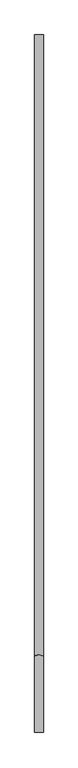
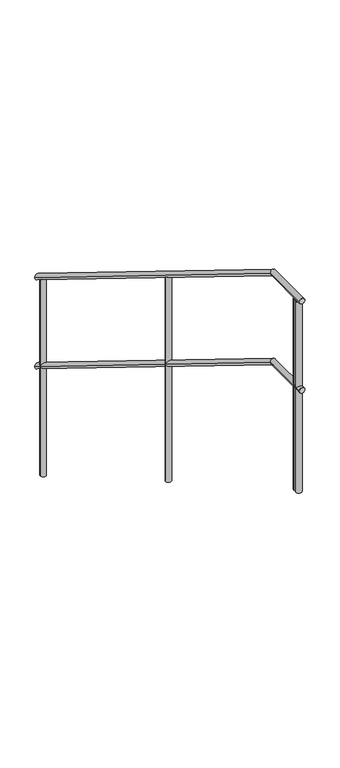
"""IFC4 building model written with IfcOpenShell, lengths in millimetres: railing geometry."""

from ifc_helpers import new_model, si_unit, point, frame, frame_2d, origin, place, context, project, spatial, circle_curve, ellipse_curve, trimmed, segment, composite_curve, outline, extrude, source, transform, mapped, element, save
from ifc_brep_helpers import plane_surface, cylinder_surface, advanced_brep


def railing_fdf8c7c9(model_context):
    return source(origin(), model_context, "Body", "SolidModel", [
        advanced_brep(
        [(-2206.0, 35476.2934796, -450.9609787), (-2176.0, 35476.2934796, -450.9609787), (-2176.0, 33312.0366941, 885.0), (-2206.0, 33312.0366941, 885.0), (-2206.0, 33046.2934796, 885.0), (-2176.0, 33046.2934796, 885.0)],
        [
            (0, 1, ellipse_curve(frame((-2191.0, 35476.2934796, -450.9609787), z_axis=(0.0, 1.0, 0.0), x_axis=(0.0, 0.0, -1.0)), 17.6276454, 15.0)),
            (1, 0, ellipse_curve(frame((-2191.0, 35476.2934796, -450.9609787), z_axis=(0.0, 1.0, 0.0), x_axis=(0.0, 0.0, -1.0)), 17.6276454, 15.0)),
            (1, 2),
            (2, 3, ellipse_curve(frame((-2191.0, 33312.0366941, 885.0), z_axis=(0.0, 0.9620125025549408, -0.27300539358770926), x_axis=(0.0, -0.27300539358770903, -0.9620125025549408)), 15.5923129, 15.0)),
            (3, 0),
            (3, 2, ellipse_curve(frame((-2191.0, 33312.0366941, 885.0), z_axis=(0.0, 0.9620125025549408, -0.27300539358770926), x_axis=(0.0, -0.27300539358770903, -0.9620125025549408)), 15.5923129, 15.0)),
            (4, 5, circle_curve(frame((-2191.0, 33046.2934796, 885.0), z_axis=(0.0, -1.0, 0.0), x_axis=(1.0, 0.0, 0.0)), 15.0)),
            (5, 4, circle_curve(frame((-2191.0, 33046.2934796, 885.0), z_axis=(0.0, -1.0, 0.0), x_axis=(1.0, 0.0, 0.0)), 15.0)),
            (2, 5),
            (4, 3),
        ],
        [
            plane_surface(frame((-2191.0, 35476.2934796, -433.3333333), z_axis=(0.0, 1.0, 0.0), x_axis=(0.0, 0.0, -1.0))),
            cylinder_surface(frame((-2191.0, 35468.4144415, -446.097375), z_axis=(0.0, 0.8509361101440399, -0.5252692037926175), x_axis=(1.0, 0.0, 0.0)), 15.0),
            plane_surface(frame((-2191.0, 33046.2934796, 900.0), z_axis=(0.0, -1.0, 0.0), x_axis=(0.0, 0.0, -1.0))),
            cylinder_surface(frame((-2191.0, 33316.2934796, 885.0), z_axis=(0.0, 1.0, 0.0), x_axis=(1.0, 0.0, 0.0)), 15.0),
        ],
        [
            (0, [[1, 2]]),
            (1, [[-2, 3, 4, 5]]),
            (1, [[-1, -5, 6, -3]]),
            (2, [[7, 8]]),
            (3, [[-4, 9, -7, 10]]),
            (3, [[-6, -10, -8, -9]]),
        ],
    ),
        advanced_brep(
        [(-2206.0, 35476.2934796, 49.0390213), (-2176.0, 35476.2934796, 49.0390213), (-2176.0, 33312.0366941, 1385.0), (-2206.0, 33312.0366941, 1385.0), (-2206.0, 33046.2934796, 1385.0), (-2176.0, 33046.2934796, 1385.0)],
        [
            (0, 1, ellipse_curve(frame((-2191.0, 35476.2934796, 49.0390213), z_axis=(0.0, 1.0, 0.0), x_axis=(0.0, 0.0, -1.0)), 17.6276454, 15.0)),
            (1, 0, ellipse_curve(frame((-2191.0, 35476.2934796, 49.0390213), z_axis=(0.0, 1.0, 0.0), x_axis=(0.0, 0.0, -1.0)), 17.6276454, 15.0)),
            (1, 2),
            (2, 3, ellipse_curve(frame((-2191.0, 33312.0366941, 1385.0), z_axis=(0.0, 0.9620125025549408, -0.27300539358770926), x_axis=(0.0, -0.27300539358770903, -0.9620125025549408)), 15.5923129, 15.0)),
            (3, 0),
            (3, 2, ellipse_curve(frame((-2191.0, 33312.0366941, 1385.0), z_axis=(0.0, 0.9620125025549408, -0.27300539358770926), x_axis=(0.0, -0.27300539358770903, -0.9620125025549408)), 15.5923129, 15.0)),
            (4, 5, circle_curve(frame((-2191.0, 33046.2934796, 1385.0), z_axis=(0.0, -1.0, 0.0), x_axis=(1.0, 0.0, 0.0)), 15.0)),
            (5, 4, circle_curve(frame((-2191.0, 33046.2934796, 1385.0), z_axis=(0.0, -1.0, 0.0), x_axis=(1.0, 0.0, 0.0)), 15.0)),
            (2, 5),
            (4, 3),
        ],
        [
            plane_surface(frame((-2191.0, 35476.2934796, 66.6666667), z_axis=(0.0, 1.0, 0.0), x_axis=(0.0, 0.0, -1.0))),
            cylinder_surface(frame((-2191.0, 35468.4144415, 53.902625), z_axis=(0.0, 0.8509361101440399, -0.5252692037926175), x_axis=(1.0, 0.0, 0.0)), 15.0),
            plane_surface(frame((-2191.0, 33046.2934796, 1400.0), z_axis=(0.0, -1.0, 0.0), x_axis=(0.0, 0.0, -1.0))),
            cylinder_surface(frame((-2191.0, 33316.2934796, 1385.0), z_axis=(0.0, 1.0, 0.0), x_axis=(1.0, 0.0, 0.0)), 15.0),
        ],
        [
            (0, [[1, 2]]),
            (1, [[-2, 3, 4, 5]]),
            (1, [[-1, -5, 6, -3]]),
            (2, [[7, 8]]),
            (3, [[-4, 9, -7, 10]]),
            (3, [[-6, -10, -8, -9]]),
        ],
    ),
        extrude(outline(composite_curve([segment(trimmed(circle_curve(frame_2d((-2191.0, 33076.2934796)), 15.0), [point((-2206.0, 33076.2934796))], [point((-2176.0, 33076.2934796))], False, "CARTESIAN"), True, "CONTINUOUS"), segment(trimmed(circle_curve(frame_2d((-2191.0, 33076.2934796)), 15.0), [point((-2176.0, 33076.2934796))], [point((-2206.0, 33076.2934796))], False, "CARTESIAN"), True, "CONTINUOUS")], self_intersect=False)), frame((0.0, 0.0, 300.0), z_axis=(0.0, 0.0, 1.0), x_axis=(1.0, 0.0, 0.0)), (0.0, 0.0, 1.0), 1070.0),
        advanced_brep(
        [(-2176.0, 34276.2934796, 777.4074074), (-2206.0, 34276.2934796, 777.4074074), (-2206.0, 34276.2934796, -366.6666667), (-2176.0, 34276.2934796, -366.6666667)],
        [
            (0, 1, ellipse_curve(frame((-2191.0, 34276.2934796, 777.4074074), z_axis=(0.0, -0.5252692037926167, -0.8509361101440406), x_axis=(0.0, -0.8509361101440406, 0.5252692037926162)), 17.6276454, 15.0)),
            (1, 2),
            (2, 3, circle_curve(frame((-2191.0, 34276.2934796, -366.6666667), z_axis=(0.0, 0.0, 1.0), x_axis=(-1.0, 0.0, 0.0)), 15.0)),
            (3, 0),
            (3, 2, circle_curve(frame((-2191.0, 34276.2934796, -366.6666667), z_axis=(0.0, 0.0, 1.0), x_axis=(-1.0, 0.0, 0.0)), 15.0)),
            (1, 0, ellipse_curve(frame((-2191.0, 34276.2934796, 777.4074074), z_axis=(0.0, -0.5252692037926167, -0.8509361101440406), x_axis=(0.0, -0.8509361101440406, 0.5252692037926162)), 17.6276454, 15.0)),
        ],
        [
            cylinder_surface(frame((-2191.0, 34276.2934796, -466.6666667), z_axis=(0.0, 0.0, 1.0), x_axis=(-1.0, 0.0, 0.0)), 15.0),
            plane_surface(frame((-2216.0, 34251.2934796, 792.8395062), z_axis=(0.0, 0.5252692037926167, 0.8509361101440406), x_axis=(1.0, 0.0, 0.0))),
            plane_surface(frame((-2216.0, 34301.2934796, -366.6666667), z_axis=(0.0, 0.0, -1.0), x_axis=(1.0, 0.0, 0.0))),
        ],
        [
            (0, [[1, 2, 3, 4]]),
            (0, [[5, -2, 6, -4]]),
            (1, [[-6, -1]]),
            (2, [[-5, -3]]),
        ],
    ),
        extrude(outline(composite_curve([segment(trimmed(circle_curve(frame_2d((-2191.0, 33096.2934796)), 15.0), [point((-2206.0, 33096.2934796))], [point((-2176.0, 33096.2934796))], False, "CARTESIAN"), True, "CONTINUOUS"), segment(trimmed(circle_curve(frame_2d((-2191.0, 33096.2934796)), 15.0), [point((-2176.0, 33096.2934796))], [point((-2206.0, 33096.2934796))], False, "CARTESIAN"), True, "CONTINUOUS")], self_intersect=False)), frame((0.0, 0.0, 300.0), z_axis=(0.0, 0.0, 1.0), x_axis=(1.0, 0.0, 0.0)), (0.0, 0.0, 1.0), 1070.0),
        advanced_brep(
        [(-2176.0, 35426.2934796, 67.5308642), (-2206.0, 35426.2934796, 67.5308642), (-2206.0, 35426.2934796, -1033.3333333), (-2176.0, 35426.2934796, -1033.3333333)],
        [
            (0, 1, ellipse_curve(frame((-2191.0, 35426.2934796, 67.5308642), z_axis=(0.0, -0.5252692037926167, -0.8509361101440406), x_axis=(0.0, -0.8509361101440406, 0.5252692037926162)), 17.6276454, 15.0)),
            (1, 2),
            (2, 3, circle_curve(frame((-2191.0, 35426.2934796, -1033.3333333), z_axis=(0.0, 0.0, 1.0), x_axis=(-1.0, 0.0, 0.0)), 15.0)),
            (3, 0),
            (3, 2, circle_curve(frame((-2191.0, 35426.2934796, -1033.3333333), z_axis=(0.0, 0.0, 1.0), x_axis=(-1.0, 0.0, 0.0)), 15.0)),
            (1, 0, ellipse_curve(frame((-2191.0, 35426.2934796, 67.5308642), z_axis=(0.0, -0.5252692037926167, -0.8509361101440406), x_axis=(0.0, -0.8509361101440406, 0.5252692037926162)), 17.6276454, 15.0)),
        ],
        [
            cylinder_surface(frame((-2191.0, 35426.2934796, -1133.3333333), z_axis=(0.0, 0.0, 1.0), x_axis=(-1.0, 0.0, 0.0)), 15.0),
            plane_surface(frame((-2216.0, 35401.2934796, 82.962963), z_axis=(0.0, 0.5252692037926167, 0.8509361101440406), x_axis=(1.0, 0.0, 0.0))),
            plane_surface(frame((-2216.0, 35451.2934796, -1033.3333333), z_axis=(0.0, 0.0, -1.0), x_axis=(1.0, 0.0, 0.0))),
        ],
        [
            (0, [[1, 2, 3, 4]]),
            (0, [[5, -2, 6, -4]]),
            (1, [[-6, -1]]),
            (2, [[-5, -3]]),
        ],
    ),
    ])


if __name__ == "__main__":
    model = new_model("IFC4")
    model_context = context("Model", 3, world=origin())
    ifc_project = project(units=[si_unit("LENGTHUNIT", "METRE", prefix="MILLI")], contexts=[model_context])
    site = spatial("IfcSite", under=ifc_project)
    building = spatial("IfcBuilding", under=site)
    placement = place(None, origin())
    railing_shape = railing_fdf8c7c9(model_context)
    element("IfcRailing", 1, at=placement, inside=building, context=model_context, shape_type="MappedRepresentation", body=[
        mapped(railing_shape, transform((0.0, 0.0, 0.0), x_axis=(1.0, 0.0, 0.0), y_axis=(0.0, 1.0, 0.0), z_axis=(0.0, 0.0, 1.0))),
    ])
    save(model, "model.ifc")
